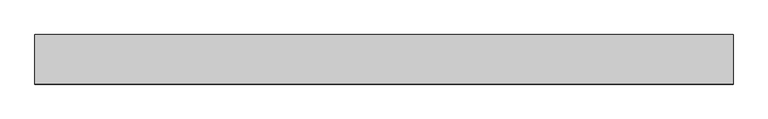
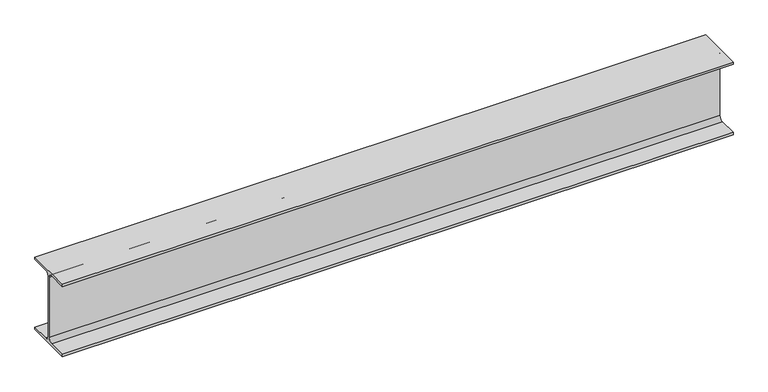
"""IFC4 building model written with IfcOpenShell, lengths in millimetres: beam geometry, 0912_Steel Framing_H-KSD3502 : H_SB_ASB_H-482x300x11x15."""

from ifc_helpers import new_model, si_unit, point, frame, frame_2d, origin, place, context, project, spatial, polyline, circle_curve, trimmed, segment, composite_curve, outline, extrude, source, transform, mapped, element, save


def beam_0ea81219(model_context):
    return source(origin(), model_context, "Body", "SweptSolid", [
        extrude(outline(composite_curve([segment(polyline([(150.0, -226.0), (150.0, -241.0), (-150.0, -241.0), (-150.0, -226.0), (-31.5, -226.0)]), True, "CONTINUOUS"), segment(trimmed(circle_curve(frame_2d((-31.5, -200.0)), 26.0), [point((-31.5, -226.0))], [point((-5.5, -200.0))], True, "CARTESIAN"), True, "CONTINUOUS"), segment(polyline([(-5.5, -200.0), (-5.5, 200.0)]), True, "CONTINUOUS"), segment(trimmed(circle_curve(frame_2d((-31.5, 200.0)), 26.0), [point((-5.5, 200.0))], [point((-31.5, 226.0))], True, "CARTESIAN"), True, "CONTINUOUS"), segment(polyline([(-31.5, 226.0), (-150.0, 226.0), (-150.0, 241.0), (150.0, 241.0), (150.0, 226.0), (31.5, 226.0)]), True, "CONTINUOUS"), segment(trimmed(circle_curve(frame_2d((31.5, 200.0)), 26.0), [point((31.5, 226.0))], [point((5.5, 200.0))], True, "CARTESIAN"), True, "CONTINUOUS"), segment(polyline([(5.5, 200.0), (5.5, -200.0)]), True, "CONTINUOUS"), segment(trimmed(circle_curve(frame_2d((31.5, -200.0)), 26.0), [point((5.5, -200.0))], [point((31.5, -226.0))], True, "CARTESIAN"), True, "CONTINUOUS"), segment(polyline([(31.5, -226.0), (150.0, -226.0)]), True, "CONTINUOUS")], self_intersect=False)), frame((-2212.3, 0.0, 0.0), z_axis=(1.0, 0.0, 0.0), x_axis=(0.0, 1.0, 0.0)), (0.0, 0.0, 1.0), 4224.6),
    ])


if __name__ == "__main__":
    model = new_model("IFC4")
    model_context = context("Model", 3, world=origin())
    ifc_project = project(units=[si_unit("LENGTHUNIT", "METRE", prefix="MILLI")], contexts=[model_context])
    site = spatial("IfcSite", under=ifc_project)
    building = spatial("IfcBuilding", under=site)
    placement = place(None, origin())
    beam_shape = beam_0ea81219(model_context)
    element("IfcBeam", 1, ObjectType="0912_Steel Framing_H-KSD3502 : H_SB_ASB_H-482x300x11x15", at=placement, inside=building, context=model_context, shape_type="MappedRepresentation", body=[
        mapped(beam_shape, transform((0.0, 0.0, 0.0), x_axis=(1.0, 0.0, 0.0), y_axis=(0.0, 1.0, 0.0), z_axis=(0.0, 0.0, 1.0))),
    ])
    save(model, "model.ifc")

# Revit data of these elements
# Type "0912_Steel Framing_H-KSD3502 : H_SB_ASB_H-482x300x11x15"
#   H_WM Code_1 = "S01AA001-00001 | Main Steel Structure Fabrication Work | Shelter/Building | Heavy Steel - Standard (Weight≥90KG/M) | Material: (   )"
#   H_WM Code_2 = "S03AA027-00001 | Main Steel Structure Erection Work | Shelter/Building | Heavy Steel (Weight≥90KG/M) | Material: (   )"
#   H_WM Code_3 = "S01AA010-00001 | Main Steel Structure Fabrication Work | Shelter/Building | Steel Painting/Coating | for Non-Fireproofed Steel Surface, Surface Preparation, Primer, Second & Final Coat | Material: (   )"
#   H_Q'ty Cal Type Tag = "SB-Q2"
#   Width = 30.0 cm
#   Web Thickness = 1.1 cm
#   Web Fillet = 2.6 cm
#   Warping Constant = 3680000.0 cm⁶
#   W = 0
#   Torsional Moment of Inertia = 88.2192 cm⁴
#   Section Area = 145.5 cm²
#   Plastic Modulus weak axis = 695.0 cm³
#   Plastic Modulus strong axis = 2790.0 cm³
#   Perimeter = 2.10 m²/m
#   Nominal Weight = 114.00 kgf/m
#   Moment of Inertia weak axis = 6760.00 cm⁴
#   Moment of Inertia strong axis = 60400.00 cm⁴
#   Height = 48.2 cm
#   Flange Thickness = 1.5 cm
#   Elastic Modulus weak axis = 451.0 cm³
#   Elastic Modulus strong axis = 2500.0 cm³
#   Centroid Vertical = 24.1 cm
#   Centroid Horizontal = 15.0 cm
#   Ix = 604000000
#   Length [instance default] = 1.5240 m
#   Zx = 2790000
#   b = 0.3000 m
#   h = 0.4820 m
#   r = 0.0260 m
#   s = 0.0110 m
#   t = 0.0150 m
#   A = 0.01455 m²
#   Structural Material [instance default] = Steel, 45-345
#   Assembly Code = ""
# Element 1 (IfcBeam, "0912_Steel Framing_H-KSD3502 : H_SB_ASB_H-482x300x11x15")
#   Structural Material = none
# Materials
#   "Steel, 45-345": class "Metal", colour RGB 189 187 185, transparency 0, Description = "Steel 345 MPa", Cost = 0
